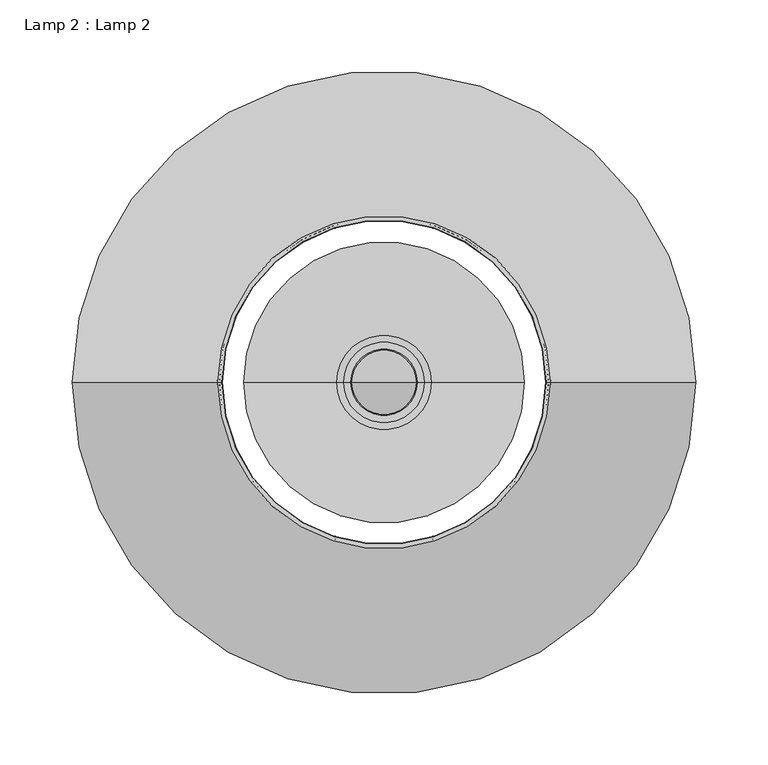
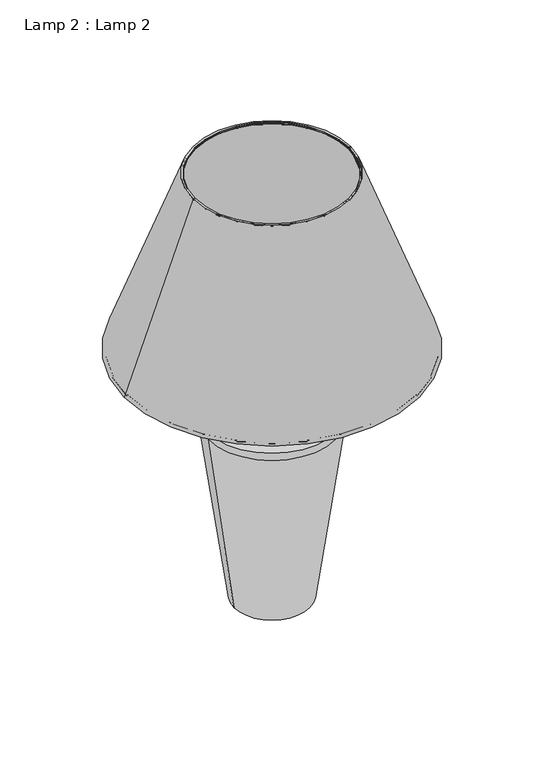
"""IFC4 building model written with IfcOpenShell, lengths in millimetres: furniture geometry, Lamp 2 : Lamp 2."""

from ifc_helpers import new_model, si_unit, point, frame, origin, place, context, project, spatial, polyline, circle_curve, ellipse_curve, trimmed, source, transform, mapped, element, save
from ifc_brep_helpers import plane_surface, cylinder_surface, revolved_surface, spline_curve, advanced_brep


def lamp_2_lamp_2_ee5345a8(model_context):
    return source(origin(), model_context, "Body", "AdvancedBrep", [
        advanced_brep(
        [(-5.625, 0.0049096, 408.6874636), (5.625, 0.0049096, 408.6874636), (5.625, 0.0049096, 396.7479044), (-5.625, 0.0049096, 396.7479044), (0.0, 0.0049096, 452.3091199), (0.0, 0.0049096, 396.7479044)],
        [
            (0, 1, circle_curve(frame((0.0, 0.0049096, 408.6874636), z_axis=(0.0, 0.0, -1.0), x_axis=(1.0, 0.0, 0.0)), 5.625)),
            (1, 2),
            (2, 3, circle_curve(frame((0.0, 0.0049096, 396.7479044), z_axis=(0.0, 0.0, 1.0), x_axis=(1.0, 0.0, 0.0)), 5.625)),
            (3, 0),
            (1, 0, circle_curve(frame((0.0, 0.0049096, 408.6874636), z_axis=(0.0, 0.0, -1.0), x_axis=(1.0, 0.0, 0.0)), 5.625)),
            (3, 2, circle_curve(frame((0.0, 0.0049096, 396.7479044), z_axis=(0.0, 0.0, 1.0), x_axis=(1.0, 0.0, 0.0)), 5.625)),
            (4, 1, circle_curve(frame((0.0, 0.0049096, 430.1356207), z_axis=(0.0, 1.0, 0.0), x_axis=(1.0, 0.0, 0.0)), 22.1734992)),
            (0, 4, circle_curve(frame((0.0, 0.0049096, 430.1356207), z_axis=(0.0, 1.0, 0.0), x_axis=(-1.0, 0.0, 0.0)), 22.1734992)),
            (2, 5),
            (5, 3),
        ],
        [
            cylinder_surface(frame((0.0, 0.0049096, 452.3091199), z_axis=(0.0, 0.0, 1.0), x_axis=(1.0, 0.0, 0.0)), 5.625),
            revolved_surface(trimmed(ellipse_curve(frame((0.0, 0.0049096, 430.1356207), z_axis=(0.0, -1.0, 0.0), x_axis=(1.0, 0.0, 0.0)), 22.1734992, 22.1734992), [point((5.625, 0.0049096, 408.6874636))], [point((0.0, 0.0049096, 452.3091199))], True, "CARTESIAN"), (0.0, 0.0049096, 452.3091199), (0.0, 0.0, 1.0)),
            plane_surface(frame((0.0, 0.0049096, 396.7479044), z_axis=(0.0, 0.0, -1.0), x_axis=(1.0, 0.0, 0.0))),
        ],
        [
            (0, [[1, 2, 3, 4]]),
            (0, [[5, -4, 6, -2]]),
            (1, [[7, -1, 8]]),
            (1, [[-8, -5, -7]]),
            (2, [[-3, 9, 10]]),
            (2, [[-6, -10, -9]]),
        ],
    ),
        advanced_brep(
        [(210.2699359, 0.0, 381.7682447), (-210.1136859, 0.0, 381.7682447), (-212.1136859, 0.0, 381.7682447), (212.2699359, 0.0, 381.7682447)],
        [
            (0, 1, circle_curve(frame((0.078125, 0.0, 381.7682447), z_axis=(0.0, 0.0, 1.0), x_axis=(-1.0, 0.0, 0.0)), 210.1918109)),
            (1, 2, circle_curve(frame((-211.1136859, 0.0, 381.7682447), z_axis=(0.0, 1.0, 0.0), x_axis=(1.0, 0.0, 0.0)), 1.0)),
            (2, 3, circle_curve(frame((0.078125, 0.0, 381.7682447), z_axis=(0.0, 0.0, -1.0), x_axis=(-1.0, 0.0, 0.0)), 212.1918109)),
            (3, 0, circle_curve(frame((211.2699359, 0.0, 381.7682447), z_axis=(0.0, 1.0, 0.0), x_axis=(-1.0, 0.0, 0.0)), 1.0)),
            (1, 0, circle_curve(frame((0.078125, 0.0, 381.7682447), z_axis=(0.0, 0.0, 1.0), x_axis=(-1.0, 0.0, 0.0)), 210.1918109)),
            (3, 2, circle_curve(frame((0.078125, 0.0, 381.7682447), z_axis=(0.0, 0.0, -1.0), x_axis=(-1.0, 0.0, 0.0)), 212.1918109)),
            (2, 1, circle_curve(frame((-211.1136859, 0.0, 381.7682447), z_axis=(0.0, 1.0, 0.0), x_axis=(1.0, 0.0, 0.0)), 1.0)),
            (0, 3, circle_curve(frame((211.2699359, 0.0, 381.7682447), z_axis=(0.0, 1.0, 0.0), x_axis=(-1.0, 0.0, 0.0)), 1.0)),
        ],
        [
            revolved_surface(trimmed(ellipse_curve(frame((-211.1136859, 0.0, 381.7682447), z_axis=(0.0, -1.0, 0.0), x_axis=(1.0, 0.0, 0.0)), 1.0, 1.0), [point((-212.1136859, 0.0, 381.7682447))], [point((-210.1136859, 0.0, 381.7682447))], True, "CARTESIAN"), (0.078125, 0.0, 370.9862512), (0.0, 0.0, -1.0)),
            revolved_surface(trimmed(ellipse_curve(frame((-211.1136859, 0.0, 381.7682447), z_axis=(0.0, -1.0, 0.0), x_axis=(1.0, 0.0, 0.0)), 1.0, 1.0), [point((-210.1136859, 0.0, 381.7682447))], [point((-212.1136859, 0.0, 381.7682447))], True, "CARTESIAN"), (0.078125, 0.0, 370.9862512), (0.0, 0.0, -1.0)),
        ],
        [
            (0, [[1, 2, 3, 4]]),
            (0, [[5, -4, 6, -2]]),
            (1, [[-3, 7, -1, 8]]),
            (1, [[-6, -8, -5, -7]]),
        ],
    ),
        advanced_brep(
        [(111.7827914, 0.0, 647.8021308), (-111.7827914, 0.0, 647.8021308), (-113.7827914, 0.0, 647.8021308), (113.7827914, 0.0, 647.8021308)],
        [
            (0, 1, circle_curve(frame((0.0, 0.0, 647.8021308), z_axis=(0.0, 0.0, 1.0), x_axis=(-1.0, 0.0, 0.0)), 111.7827914)),
            (1, 2, circle_curve(frame((-112.7827914, 0.0, 647.8021308), z_axis=(0.0, 1.0, 0.0), x_axis=(1.0, 0.0, 0.0)), 1.0)),
            (2, 3, circle_curve(frame((0.0, 0.0, 647.8021308), z_axis=(0.0, 0.0, -1.0), x_axis=(-1.0, 0.0, 0.0)), 113.7827914)),
            (3, 0, circle_curve(frame((112.7827914, 0.0, 647.8021308), z_axis=(0.0, 1.0, 0.0), x_axis=(-1.0, 0.0, 0.0)), 1.0)),
            (1, 0, circle_curve(frame((0.0, 0.0, 647.8021308), z_axis=(0.0, 0.0, 1.0), x_axis=(-1.0, 0.0, 0.0)), 111.7827914)),
            (3, 2, circle_curve(frame((0.0, 0.0, 647.8021308), z_axis=(0.0, 0.0, -1.0), x_axis=(-1.0, 0.0, 0.0)), 113.7827914)),
            (2, 1, circle_curve(frame((-112.7827914, 0.0, 647.8021308), z_axis=(0.0, 1.0, 0.0), x_axis=(1.0, 0.0, 0.0)), 1.0)),
            (0, 3, circle_curve(frame((112.7827914, 0.0, 647.8021308), z_axis=(0.0, 1.0, 0.0), x_axis=(-1.0, 0.0, 0.0)), 1.0)),
        ],
        [
            revolved_surface(trimmed(ellipse_curve(frame((-112.7827914, 0.0, 647.8021308), z_axis=(0.0, -1.0, 0.0), x_axis=(1.0, 0.0, 0.0)), 1.0, 1.0), [point((-113.7827914, 0.0, 647.8021308))], [point((-111.7827914, 0.0, 647.8021308))], True, "CARTESIAN"), (0.0, 0.0, 669.21875), (0.0, 0.0, -1.0)),
            revolved_surface(trimmed(ellipse_curve(frame((-112.7827914, 0.0, 647.8021308), z_axis=(0.0, -1.0, 0.0), x_axis=(1.0, 0.0, 0.0)), 1.0, 1.0), [point((-111.7827914, 0.0, 647.8021308))], [point((-113.7827914, 0.0, 647.8021308))], True, "CARTESIAN"), (0.0, 0.0, 669.21875), (0.0, 0.0, -1.0)),
        ],
        [
            (0, [[1, 2, 3, 4]]),
            (0, [[5, -4, 6, -2]]),
            (1, [[-3, 7, -1, 8]]),
            (1, [[-6, -8, -5, -7]]),
        ],
    ),
        advanced_brep(
        [(0.0, 0.0, 380.0), (-32.5, 0.0, 380.0), (32.5, 0.0, 380.0), (10.0478847, 0.0, 406.8452028), (-10.0478847, 0.0, 406.8452028), (0.0, 0.0, 406.8452028), (7.1801044, 0.0, 396.1425012), (-7.1801044, 0.0, 396.1425012), (8.4301044, 0.0, 396.1425012), (-8.4301044, 0.0, 396.1425012), (13.1200696, 0.0, 393.7368661), (-13.1200696, 0.0, 393.7368661), (13.1200696, 0.0, 390.7616675), (-13.1200696, 0.0, 390.7616675), (18.1200696, 0.0, 390.7616675), (-18.1200696, 0.0, 390.7616675), (22.8100348, 0.0, 388.3560323), (-22.8100348, 0.0, 388.3560323), (22.8100348, 0.0, 385.3808337), (-22.8100348, 0.0, 385.3808337), (27.8100348, 0.0, 385.3808337), (-27.8100348, 0.0, 385.3808337), (32.5, 0.0, 382.9751986), (-32.5, 0.0, 382.9751986)],
        [
            (0, 1),
            (1, 2, circle_curve(frame((0.0, 0.0, 380.0), z_axis=(0.0, 0.0, -1.0), x_axis=(-1.0, 0.0, 0.0)), 32.5)),
            (2, 0),
            (2, 1, circle_curve(frame((0.0, 0.0, 380.0), z_axis=(0.0, 0.0, -1.0), x_axis=(-1.0, 0.0, 0.0)), 32.5)),
            (3, 4, circle_curve(frame((0.0, 0.0, 406.8452028), z_axis=(0.0, 0.0, 1.0), x_axis=(-1.0, 0.0, 0.0)), 10.0478847)),
            (4, 5),
            (5, 3),
            (4, 3, circle_curve(frame((0.0, 0.0, 406.8452028), z_axis=(0.0, 0.0, 1.0), x_axis=(-1.0, 0.0, 0.0)), 10.0478847)),
            (6, 7, circle_curve(frame((0.0, 0.0, 396.1425012), z_axis=(0.0, 0.0, 1.0), x_axis=(-1.0, 0.0, 0.0)), 7.1801044)),
            (7, 4),
            (3, 6),
            (7, 6, circle_curve(frame((0.0, 0.0, 396.1425012), z_axis=(0.0, 0.0, 1.0), x_axis=(-1.0, 0.0, 0.0)), 7.1801044)),
            (8, 9, circle_curve(frame((0.0, 0.0, 396.1425012), z_axis=(0.0, 0.0, 1.0), x_axis=(-1.0, 0.0, 0.0)), 8.4301044)),
            (9, 7),
            (6, 8),
            (9, 8, circle_curve(frame((0.0, 0.0, 396.1425012), z_axis=(0.0, 0.0, 1.0), x_axis=(-1.0, 0.0, 0.0)), 8.4301044)),
            (10, 11, circle_curve(frame((0.0, 0.0, 393.7368661), z_axis=(0.0, 0.0, 1.0), x_axis=(-1.0, 0.0, 0.0)), 13.1200696)),
            (11, 9, circle_curve(frame((-7.7356139, 0.0, 389.0140039), z_axis=(0.0, 1.0, 0.0), x_axis=(1.0, 0.0, 0.0)), 7.1622476)),
            (8, 10, circle_curve(frame((7.7356139, 0.0, 389.0140039), z_axis=(0.0, 1.0, 0.0), x_axis=(-1.0, 0.0, 0.0)), 7.1622476)),
            (11, 10, circle_curve(frame((0.0, 0.0, 393.7368661), z_axis=(0.0, 0.0, 1.0), x_axis=(-1.0, 0.0, 0.0)), 13.1200696)),
            (12, 13, circle_curve(frame((0.0, 0.0, 390.7616675), z_axis=(0.0, 0.0, 1.0), x_axis=(-1.0, 0.0, 0.0)), 13.1200696)),
            (13, 11),
            (10, 12),
            (13, 12, circle_curve(frame((0.0, 0.0, 390.7616675), z_axis=(0.0, 0.0, 1.0), x_axis=(-1.0, 0.0, 0.0)), 13.1200696)),
            (14, 15, circle_curve(frame((0.0, 0.0, 390.7616675), z_axis=(0.0, 0.0, 1.0), x_axis=(-1.0, 0.0, 0.0)), 18.1200696)),
            (15, 13),
            (12, 14),
            (15, 14, circle_curve(frame((0.0, 0.0, 390.7616675), z_axis=(0.0, 0.0, 1.0), x_axis=(-1.0, 0.0, 0.0)), 18.1200696)),
            (16, 17, circle_curve(frame((0.0, 0.0, 388.3560323), z_axis=(0.0, 0.0, 1.0), x_axis=(-1.0, 0.0, 0.0)), 22.8100348)),
            (17, 15, circle_curve(frame((-17.4255791, 0.0, 383.6331702), z_axis=(0.0, 1.0, 0.0), x_axis=(1.0, 0.0, 0.0)), 7.1622476)),
            (14, 16, circle_curve(frame((17.4255791, 0.0, 383.6331702), z_axis=(0.0, 1.0, 0.0), x_axis=(-1.0, 0.0, 0.0)), 7.1622476)),
            (17, 16, circle_curve(frame((0.0, 0.0, 388.3560323), z_axis=(0.0, 0.0, 1.0), x_axis=(-1.0, 0.0, 0.0)), 22.8100348)),
            (18, 19, circle_curve(frame((0.0, 0.0, 385.3808337), z_axis=(0.0, 0.0, 1.0), x_axis=(-1.0, 0.0, 0.0)), 22.8100348)),
            (19, 17),
            (16, 18),
            (19, 18, circle_curve(frame((0.0, 0.0, 385.3808337), z_axis=(0.0, 0.0, 1.0), x_axis=(-1.0, 0.0, 0.0)), 22.8100348)),
            (20, 21, circle_curve(frame((0.0, 0.0, 385.3808337), z_axis=(0.0, 0.0, 1.0), x_axis=(-1.0, 0.0, 0.0)), 27.8100348)),
            (21, 19),
            (18, 20),
            (21, 20, circle_curve(frame((0.0, 0.0, 385.3808337), z_axis=(0.0, 0.0, 1.0), x_axis=(-1.0, 0.0, 0.0)), 27.8100348)),
            (22, 23, circle_curve(frame((0.0, 0.0, 382.9751986), z_axis=(0.0, 0.0, 1.0), x_axis=(-1.0, 0.0, 0.0)), 32.5)),
            (23, 21, circle_curve(frame((-27.1155443, 0.0, 378.2523365), z_axis=(0.0, 1.0, 0.0), x_axis=(1.0, 0.0, 0.0)), 7.1622476)),
            (20, 22, circle_curve(frame((27.1155443, 0.0, 378.2523365), z_axis=(0.0, 1.0, 0.0), x_axis=(-1.0, 0.0, 0.0)), 7.1622476)),
            (23, 22, circle_curve(frame((0.0, 0.0, 382.9751986), z_axis=(0.0, 0.0, 1.0), x_axis=(-1.0, 0.0, 0.0)), 32.5)),
            (1, 23),
            (22, 2),
        ],
        [
            plane_surface(frame((0.0, 0.0, 380.0), z_axis=(0.0, 0.0, -1.0), x_axis=(-1.0, 0.0, 0.0))),
            plane_surface(frame((0.0, 0.0, 406.8452028), z_axis=(0.0, 0.0, 1.0), x_axis=(-1.0, 0.0, 0.0))),
            revolved_surface(polyline([(-10.0478847, 0.0, 406.8452028), (-7.1801044, 0.0, 396.1425012)]), (0.0, 0.0, 417.9746199), (0.0, 0.0, -1.0)),
            plane_surface(frame((0.0, 0.0, 396.1425012), z_axis=(0.0, 0.0, 1.0), x_axis=(-1.0, 0.0, 0.0))),
            revolved_surface(trimmed(ellipse_curve(frame((-7.7356139, 0.0, 389.0140039), z_axis=(0.0, -1.0, 0.0), x_axis=(1.0, 0.0, 0.0)), 7.1622476, 7.1622476), [point((-8.4301044, 0.0, 396.1425012))], [point((-13.1200696, 0.0, 393.7368661))], True, "CARTESIAN"), (0.0, 0.0, 417.9746199), (0.0, 0.0, -1.0)),
            cylinder_surface(frame((0.0, 0.0, 417.9746199), z_axis=(0.0, 0.0, -1.0), x_axis=(-1.0, 0.0, 0.0)), 13.1200696),
            plane_surface(frame((0.0, 0.0, 390.7616675), z_axis=(0.0, 0.0, 1.0), x_axis=(-1.0, 0.0, 0.0))),
            revolved_surface(trimmed(ellipse_curve(frame((-17.4255791, 0.0, 383.6331702), z_axis=(0.0, -1.0, 0.0), x_axis=(1.0, 0.0, 0.0)), 7.1622476, 7.1622476), [point((-18.1200696, 0.0, 390.7616675))], [point((-22.8100348, 0.0, 388.3560323))], True, "CARTESIAN"), (0.0, 0.0, 417.9746199), (0.0, 0.0, -1.0)),
            cylinder_surface(frame((0.0, 0.0, 417.9746199), z_axis=(0.0, 0.0, -1.0), x_axis=(-1.0, 0.0, 0.0)), 22.8100348),
            plane_surface(frame((0.0, 0.0, 385.3808337), z_axis=(0.0, 0.0, 1.0), x_axis=(-1.0, 0.0, 0.0))),
            revolved_surface(trimmed(ellipse_curve(frame((-27.1155443, 0.0, 378.2523365), z_axis=(0.0, -1.0, 0.0), x_axis=(1.0, 0.0, 0.0)), 7.1622476, 7.1622476), [point((-27.8100348, 0.0, 385.3808337))], [point((-32.5, 0.0, 382.9751986))], True, "CARTESIAN"), (0.0, 0.0, 417.9746199), (0.0, 0.0, -1.0)),
            cylinder_surface(frame((0.0, 0.0, 417.9746199), z_axis=(0.0, 0.0, -1.0), x_axis=(-1.0, 0.0, 0.0)), 32.5),
        ],
        [
            (0, [[1, 2, 3]]),
            (0, [[-3, 4, -1]]),
            (1, [[5, 6, 7]]),
            (1, [[8, -7, -6]]),
            (2, [[9, 10, -5, 11]]),
            (2, [[12, -11, -8, -10]]),
            (3, [[13, 14, -9, 15]]),
            (3, [[16, -15, -12, -14]]),
            (4, [[17, 18, -13, 19]]),
            (4, [[20, -19, -16, -18]]),
            (5, [[21, 22, -17, 23]]),
            (5, [[24, -23, -20, -22]]),
            (6, [[25, 26, -21, 27]]),
            (6, [[28, -27, -24, -26]]),
            (7, [[29, 30, -25, 31]]),
            (7, [[32, -31, -28, -30]]),
            (8, [[33, 34, -29, 35]]),
            (8, [[36, -35, -32, -34]]),
            (9, [[37, 38, -33, 39]]),
            (9, [[40, -39, -36, -38]]),
            (10, [[41, 42, -37, 43]]),
            (10, [[44, -43, -40, -42]]),
            (11, [[-2, 45, -41, 46]]),
            (11, [[-4, -46, -44, -45]]),
        ],
    ),
        advanced_brep(
        [(55.0, 0.0, 0.0), (-55.0, 0.0, 0.0), (-93.2726028, 0.0, 272.3237189), (93.2726028, 0.0, 272.3237189), (0.0, 0.0, 0.0), (32.5, 0.0, 380.0), (-32.5, 0.0, 380.0), (0.0, 0.0, 380.0), (95.0446085, 0.0, 284.932195), (-95.0446085, 0.0, 284.932195)],
        [
            (0, 1, circle_curve(frame((0.0, 0.0, 0.0), z_axis=(0.0, 0.0, 1.0), x_axis=(-1.0, 0.0, 0.0)), 55.0)),
            (1, 2),
            (2, 3, circle_curve(frame((0.0, 0.0, 272.3237189), z_axis=(0.0, 0.0, -1.0), x_axis=(-1.0, 0.0, 0.0)), 93.2726028)),
            (3, 0),
            (1, 0, circle_curve(frame((0.0, 0.0, 0.0), z_axis=(0.0, 0.0, 1.0), x_axis=(-1.0, 0.0, 0.0)), 55.0)),
            (3, 2, circle_curve(frame((0.0, 0.0, 272.3237189), z_axis=(0.0, 0.0, -1.0), x_axis=(-1.0, 0.0, 0.0)), 93.2726028)),
            (4, 1),
            (0, 4),
            (5, 6, circle_curve(frame((0.0, 0.0, 380.0), z_axis=(0.0, 0.0, 1.0), x_axis=(-1.0, 0.0, 0.0)), 32.5)),
            (6, 7),
            (7, 5),
            (6, 5, circle_curve(frame((0.0, 0.0, 380.0), z_axis=(0.0, 0.0, 1.0), x_axis=(-1.0, 0.0, 0.0)), 32.5)),
            (8, 9, circle_curve(frame((0.0, 0.0, 284.932195), z_axis=(0.0, 0.0, 1.0), x_axis=(-1.0, 0.0, 0.0)), 95.0446085)),
            (9, 6, spline_curve(3, [(-95.0446085, 0.0, 284.932195), (-97.453949935, 0.0, 298.596249282), (-96.188694178, 0.0, 303.810562504), (-91.4761635, 0.0, 311.111813345), (-87.982441251, 0.0, 313.128914852), (-80.007669597, 0.0, 317.691178928), (-75.616399887, 0.0, 320.187545578), (-71.996617923, 0.0, 325.651073111), (-71.996617881, 0.0, 328.458469354), (-71.615996393, 0.0, 332.724687482), (-71.353175804, 0.0, 334.331973474), (-70.786475665, 0.0, 337.797642111), (-70.481715894, 0.0, 339.661407947), (-71.254006942, 0.0, 343.624329421), (-72.504543085, 0.0, 345.724406697), (-76.143249721, 0.0, 350.099491704), (-78.742373361, 0.0, 351.600096459), (-86.562175204, 0.0, 356.114861157), (-92.020074445, 0.0, 359.265980803), (-98.470606982, 0.0, 366.885189171), (-97.195457616, 0.0, 371.424256987), (-88.6243529, 0.0, 376.130489061), (-81.983535995, 0.0, 376.711485228), (-67.143390223, 0.0, 378.570660036), (-59.037200537, 0.0, 380.0), (-32.5, 0.0, 380.0)], [4, 2, 2, 2, 2, 2, 2, 2, 2, 2, 2, 2, 4], [0.0, 0.03985914919293754, 0.08057749635778949, 0.11834827401611286, 0.14948322781927886, 0.17098203520545735, 0.19303228957060214, 0.21777825276599289, 0.2586170795711167, 0.30356033835425955, 0.3644303221319498, 0.4188228813927918, 0.48866624030450706])),
            (5, 8, spline_curve(3, [(32.5, 0.0, 380.0), (59.037200537, 0.0, 380.0), (67.143390223, 0.0, 378.570660036), (81.983535995, 0.0, 376.711485228), (88.6243529, 0.0, 376.130489061), (97.195457616, 0.0, 371.424256987), (98.470606982, 0.0, 366.885189171), (92.020074445, 0.0, 359.265980803), (86.562175204, 0.0, 356.114861157), (78.742373361, 0.0, 351.600096459), (76.143249721, 0.0, 350.099491704), (72.504543085, 0.0, 345.724406697), (71.254006942, 0.0, 343.624329421), (70.481715894, 0.0, 339.661407947), (70.786475665, 0.0, 337.797642111), (71.353175804, 0.0, 334.331973474), (71.615996393, 0.0, 332.724687482), (71.996617881, 0.0, 328.458469354), (71.996617923, 0.0, 325.651073111), (75.616399887, 0.0, 320.187545578), (80.007669597, 0.0, 317.691178928), (87.982441251, 0.0, 313.128914852), (91.4761635, 0.0, 311.111813345), (96.188694178, 0.0, 303.810562504), (97.453949935, 0.0, 298.596249282), (95.0446085, 0.0, 284.932195)], [4, 2, 2, 2, 2, 2, 2, 2, 2, 2, 2, 2, 4], [0.0, 0.06984335891171527, 0.12423591817255722, 0.1851059019502475, 0.23004916073339038, 0.2708879875385142, 0.2956339507339049, 0.3176842050990497, 0.3391830124852282, 0.3703179662883942, 0.40808874394671757, 0.4488070911115695, 0.48866624030450706])),
            (9, 8, circle_curve(frame((0.0, 0.0, 284.932195), z_axis=(0.0, 0.0, 1.0), x_axis=(-1.0, 0.0, 0.0)), 95.0446085)),
            (2, 9),
            (8, 3),
        ],
        [
            revolved_surface(polyline([(-93.2726028, 0.0, 272.3237189), (-55.0, 0.0, 0.0)]), (0.0, 0.0, 420.0), (0.0, 0.0, -1.0)),
            plane_surface(frame((0.0, 0.0, 0.0), z_axis=(0.0, 0.0, -1.0), x_axis=(-1.0, 0.0, 0.0))),
            plane_surface(frame((0.0, 0.0, 380.0), z_axis=(0.0, 0.0, 1.0), x_axis=(-1.0, 0.0, 0.0))),
            revolved_surface(spline_curve(3, [(-32.5, 0.0, 380.0), (-59.037200537, 0.0, 380.0), (-67.143390223, 0.0, 378.570660036), (-81.983535995, 0.0, 376.711485228), (-88.6243529, 0.0, 376.130489061), (-97.195457616, 0.0, 371.424256987), (-98.470606982, 0.0, 366.885189171), (-92.020074445, 0.0, 359.265980803), (-86.562175204, 0.0, 356.114861157), (-78.742373361, 0.0, 351.600096459), (-76.143249721, 0.0, 350.099491704), (-72.504543085, 0.0, 345.724406697), (-71.254006942, 0.0, 343.624329421), (-70.481715894, 0.0, 339.661407947), (-70.786475665, 0.0, 337.797642111), (-71.353175804, 0.0, 334.331973474), (-71.615996393, 0.0, 332.724687482), (-71.996617881, 0.0, 328.458469354), (-71.996617923, 0.0, 325.651073111), (-75.616399887, 0.0, 320.187545578), (-80.007669597, 0.0, 317.691178928), (-87.982441251, 0.0, 313.128914852), (-91.4761635, 0.0, 311.111813345), (-96.188694178, 0.0, 303.810562504), (-97.453949935, 0.0, 298.596249282), (-95.0446085, 0.0, 284.932195)], [4, 2, 2, 2, 2, 2, 2, 2, 2, 2, 2, 2, 4], [0.0, 0.06984335891171527, 0.12423591817255722, 0.1851059019502475, 0.23004916073339038, 0.2708879875385142, 0.2956339507339049, 0.3176842050990497, 0.3391830124852282, 0.3703179662883942, 0.40808874394671757, 0.4488070911115695, 0.48866624030450706]), (0.0, 0.0, 420.0), (0.0, 0.0, -1.0)),
            revolved_surface(polyline([(-95.0446085, 0.0, 284.932195), (-93.2726028, 0.0, 272.3237189)]), (0.0, 0.0, 420.0), (0.0, 0.0, -1.0)),
        ],
        [
            (0, [[1, 2, 3, 4]]),
            (0, [[5, -4, 6, -2]]),
            (1, [[7, -1, 8]]),
            (1, [[-8, -5, -7]]),
            (2, [[9, 10, 11]]),
            (2, [[12, -11, -10]]),
            (3, [[13, 14, -9, 15]]),
            (3, [[16, -15, -12, -14]]),
            (4, [[-3, 17, -13, 18]]),
            (4, [[-6, -18, -16, -17]]),
        ],
    ),
        advanced_brep(
        [(-115.0, 0.0, 650.0), (115.0, 0.0, 650.0), (215.0, 0.0, 380.0), (-215.0, 0.0, 380.0), (-111.9695243, 0.0, 650.0), (111.9695243, 0.0, 650.0), (-212.7058705, 0.0, 380.7941496), (212.7058705, 0.0, 380.7941496), (113.4388971, 0.0, 648.8149779), (-113.4388971, 0.0, 648.8149779), (211.2249908, 0.0, 380.0), (-211.2249908, 0.0, 380.0), (-111.9695243, 0.0, 648.8149779), (111.9695243, 0.0, 648.8149779), (-211.2249908, 0.0, 380.7941496), (211.2249908, 0.0, 380.7941496)],
        [
            (0, 1, circle_curve(frame((0.0, 0.0, 650.0), z_axis=(0.0, 0.0, -1.0), x_axis=(1.0, 0.0, 0.0)), 115.0)),
            (1, 2),
            (2, 3, circle_curve(frame((0.0, 0.0, 380.0), z_axis=(0.0, 0.0, 1.0), x_axis=(1.0, 0.0, 0.0)), 215.0)),
            (3, 0),
            (1, 0, circle_curve(frame((0.0, 0.0, 650.0), z_axis=(0.0, 0.0, -1.0), x_axis=(1.0, 0.0, 0.0)), 115.0)),
            (3, 2, circle_curve(frame((0.0, 0.0, 380.0), z_axis=(0.0, 0.0, 1.0), x_axis=(1.0, 0.0, 0.0)), 215.0)),
            (4, 5, circle_curve(frame((0.0, 0.0, 650.0), z_axis=(0.0, 0.0, -1.0), x_axis=(1.0, 0.0, 0.0)), 111.9695243)),
            (5, 1),
            (0, 4),
            (5, 4, circle_curve(frame((0.0, 0.0, 650.0), z_axis=(0.0, 0.0, -1.0), x_axis=(1.0, 0.0, 0.0)), 111.9695243)),
            (6, 7, circle_curve(frame((0.0, 0.0, 380.7941496), z_axis=(0.0, 0.0, -1.0), x_axis=(1.0, 0.0, 0.0)), 212.7058705)),
            (7, 8),
            (8, 9, circle_curve(frame((0.0, 0.0, 648.8149779), z_axis=(0.0, 0.0, 1.0), x_axis=(1.0, 0.0, 0.0)), 113.4388971)),
            (9, 6),
            (7, 6, circle_curve(frame((0.0, 0.0, 380.7941496), z_axis=(0.0, 0.0, -1.0), x_axis=(1.0, 0.0, 0.0)), 212.7058705)),
            (9, 8, circle_curve(frame((0.0, 0.0, 648.8149779), z_axis=(0.0, 0.0, 1.0), x_axis=(1.0, 0.0, 0.0)), 113.4388971)),
            (2, 10),
            (10, 11, circle_curve(frame((0.0, 0.0, 380.0), z_axis=(0.0, 0.0, 1.0), x_axis=(1.0, 0.0, 0.0)), 211.2249908)),
            (11, 3),
            (11, 10, circle_curve(frame((0.0, 0.0, 380.0), z_axis=(0.0, 0.0, 1.0), x_axis=(1.0, 0.0, 0.0)), 211.2249908)),
            (12, 13, circle_curve(frame((0.0, 0.0, 648.8149779), z_axis=(0.0, 0.0, -1.0), x_axis=(1.0, 0.0, 0.0)), 111.9695243)),
            (13, 5),
            (4, 12),
            (13, 12, circle_curve(frame((0.0, 0.0, 648.8149779), z_axis=(0.0, 0.0, -1.0), x_axis=(1.0, 0.0, 0.0)), 111.9695243)),
            (8, 13),
            (12, 9),
            (14, 15, circle_curve(frame((0.0, 0.0, 380.7941496), z_axis=(0.0, 0.0, -1.0), x_axis=(1.0, 0.0, 0.0)), 211.2249908)),
            (15, 7),
            (6, 14),
            (15, 14, circle_curve(frame((0.0, 0.0, 380.7941496), z_axis=(0.0, 0.0, -1.0), x_axis=(1.0, 0.0, 0.0)), 211.2249908)),
            (10, 15),
            (14, 11),
        ],
        [
            revolved_surface(polyline([(215.0, 0.0, 380.0), (115.0, 0.0, 650.0)]), (0.0, 0.0, 690.0), (0.0, 0.0, 1.0)),
            plane_surface(frame((0.0, 0.0, 650.0), z_axis=(0.0, 0.0, 1.0), x_axis=(1.0, 0.0, 0.0))),
            revolved_surface(polyline([(113.4388971, 0.0, 648.8149779), (212.7058705, 0.0, 380.7941496)]), (0.0, 0.0, 690.0), (0.0, 0.0, 1.0)),
            plane_surface(frame((0.0, 0.0, 380.0), z_axis=(0.0, 0.0, -1.0), x_axis=(1.0, 0.0, 0.0))),
            revolved_surface(polyline([(111.9695243, 0.0, 650.0), (111.9695243, 0.0, 648.8149779)]), (0.0, 0.0, 690.0), (0.0, 0.0, 1.0)),
            plane_surface(frame((0.0, 0.0, 648.8149779), z_axis=(0.0, 0.0, -1.0), x_axis=(1.0, 0.0, 0.0))),
            plane_surface(frame((0.0, 0.0, 380.7941496), z_axis=(0.0, 0.0, 1.0), x_axis=(1.0, 0.0, 0.0))),
            revolved_surface(polyline([(211.2249908, 0.0, 380.7941496), (211.2249908, 0.0, 380.0)]), (0.0, 0.0, 690.0), (0.0, 0.0, 1.0)),
        ],
        [
            (0, [[1, 2, 3, 4]]),
            (0, [[5, -4, 6, -2]]),
            (1, [[7, 8, -1, 9]]),
            (1, [[10, -9, -5, -8]]),
            (2, [[11, 12, 13, 14]]),
            (2, [[15, -14, 16, -12]]),
            (3, [[-3, 17, 18, 19]]),
            (3, [[-6, -19, 20, -17]]),
            (4, [[21, 22, -7, 23]]),
            (4, [[24, -23, -10, -22]]),
            (5, [[-13, 25, -21, 26]]),
            (5, [[-16, -26, -24, -25]]),
            (6, [[27, 28, -11, 29]]),
            (6, [[30, -29, -15, -28]]),
            (7, [[-18, 31, -27, 32]]),
            (7, [[-20, -32, -30, -31]]),
        ],
    ),
    ])


if __name__ == "__main__":
    model = new_model("IFC4")
    model_context = context("Model", 3, world=origin())
    ifc_project = project(units=[si_unit("LENGTHUNIT", "METRE", prefix="MILLI")], contexts=[model_context])
    site = spatial("IfcSite", under=ifc_project)
    building = spatial("IfcBuilding", under=site)
    placement = place(None, origin())
    lamp_2_lamp_2_shape = lamp_2_lamp_2_ee5345a8(model_context)
    element("IfcFurniture", 1, ObjectType="Lamp 2 : Lamp 2", at=placement, inside=building, context=model_context, shape_type="MappedRepresentation", body=[
        mapped(lamp_2_lamp_2_shape, transform((0.0, 0.0, 0.0), x_axis=(1.0, 0.0, 0.0), y_axis=(0.0, 1.0, 0.0), z_axis=(0.0, 0.0, 1.0))),
    ])
    save(model, "model.ifc")

# Revit data of these elements
# Type "Lamp 2 : Lamp 2"
#   Default Elevation = 0
# Element 1 (IfcFurniture, "Lamp 2 : Lamp 2")
#   Materials on its faces: "Thermoplastic Resin", "Fabric Lamp Shade", "Default New Material", "Default Light Source"
# Materials
#   "Thermoplastic Resin": class "Plastic", colour RGB 255 255 125, transparency 0, Description = "Thermoplastic Resin", Cost = 0
#   "Fabric Lamp Shade": class "Generic", colour RGB 118 184 128, transparency 0.51, Cost = 0
#   "Default New Material": class "Generic", colour RGB 151 217 182, transparency 0, Description = "Porcelin", Cost = 0
#   "Default Light Source": class "System", colour RGB 255 255 0, transparency 0.75, Comments = "Rendering appearance not upgraded "
